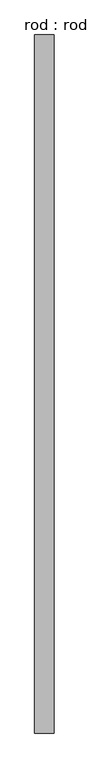
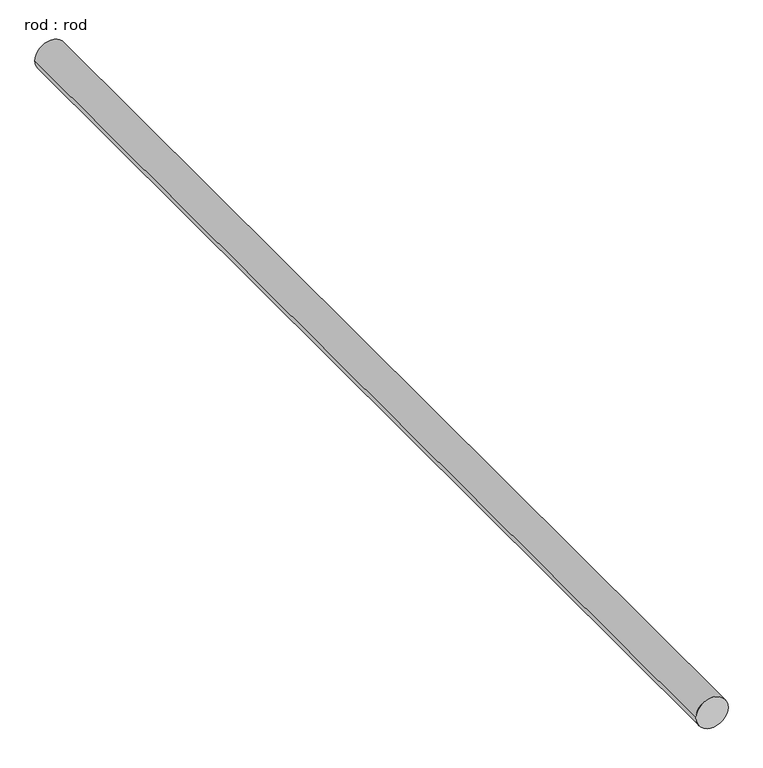
"""IFC4 building model written with IfcOpenShell, lengths in millimetres: proxy geometry, rod : rod."""

import ifcopenshell
import ifcopenshell.guid

model = None  # the IFC model being written
_history = None  # IfcOwnerHistory: only IFC2X3 demands one
_inside = {}  # id of a spatial element -> (the spatial element, [elements in it])
_under = {}  # id of a project, library or spatial element -> (it, [spatial elements below it])
_declared = {}  # id of a project -> (the project, [libraries it declares])
_typed = {}  # id of a type object -> (the type object, [elements of that type])
_made_of = {}  # id of a material, layer set ... -> (it, [elements and type objects made of it])


def new_model(schema):
    """Start an empty IFC model of exactly this schema.

    Asked for "IFC4X3", IfcOpenShell would pick the latest addendum, in which some entities
    have other attributes; the version numbers below select the first issue.
    IFC2X3 requires an IfcOwnerHistory on every rooted entity: one is made here for all.
    """
    global model, _history
    if schema == "IFC4X3":
        model = ifcopenshell.file(schema_version=(4, 3, 0, 0))
    else:
        model = ifcopenshell.file(schema=schema)
    _inside.clear()
    _under.clear()
    _declared.clear()
    _typed.clear()
    _made_of.clear()
    _history = None
    if model.schema == "IFC2X3":
        org = make("IfcOrganization", Name="unknown")
        user = make(
            "IfcPersonAndOrganization",
            ThePerson=make("IfcPerson", FamilyName="unknown"),
            TheOrganization=org,
        )
        app = make(
            "IfcApplication",
            ApplicationDeveloper=org,
            Version="unknown",
            ApplicationFullName="unknown",
            ApplicationIdentifier="unknown",
        )
        _history = make(
            "IfcOwnerHistory",
            OwningUser=user,
            OwningApplication=app,
            ChangeAction="ADDED",
            CreationDate=0,
        )
    return model


def make(cls, **values):
    """One entity of the class cls with the attributes given. An attribute that is None is left unset."""
    return model.create_entity(
        cls, **{name: value for name, value in values.items() if value is not None}
    )


def rooted(cls, **values):
    """An entity with a GlobalId (a new one), such as an element, a storey or a relation."""
    return make(cls, GlobalId=ifcopenshell.guid.new(), OwnerHistory=_history, **values)


def si_unit(unit_type, name, prefix=None):
    """IfcSIUnit, for example si_unit("LENGTHUNIT", "METRE", prefix="MILLI")."""
    return make("IfcSIUnit", UnitType=unit_type, Prefix=prefix, Name=name)


def assignment(units):
    """IfcUnitAssignment: the units of a project."""
    return None if units is None else make("IfcUnitAssignment", Units=units)


def point(xyz):
    """IfcCartesianPoint."""
    return None if xyz is None else make("IfcCartesianPoint", Coordinates=xyz)


def direction(xyz):
    """IfcDirection."""
    return None if xyz is None else make("IfcDirection", DirectionRatios=xyz)


def frame(location, z_axis=None, x_axis=None):
    """IfcAxis2Placement3D, a coordinate frame: its origin and axes. An axis left out is left unset."""
    return make(
        "IfcAxis2Placement3D",
        Location=point(location),
        Axis=direction(z_axis),
        RefDirection=direction(x_axis),
    )


def frame_2d(location, x_axis=None):
    """IfcAxis2Placement2D, a coordinate frame in the plane: its origin and x axis."""
    return make(
        "IfcAxis2Placement2D", Location=point(location), RefDirection=direction(x_axis)
    )


def origin():
    """The frame at (0, 0, 0) with its axes left unset."""
    return frame((0.0, 0.0, 0.0))


def place(relative_to, where):
    """IfcLocalPlacement: puts the frame where relative to a parent placement (None: the world)."""
    return make(
        "IfcLocalPlacement", PlacementRelTo=relative_to, RelativePlacement=where
    )


def context(
    kind, dimensions, precision=None, world=None, true_north=None, identifier=None
):
    """IfcGeometricRepresentationContext, for example the 3D "Model" context."""
    return make(
        "IfcGeometricRepresentationContext",
        ContextIdentifier=identifier,
        ContextType=kind,
        CoordinateSpaceDimension=dimensions,
        Precision=precision,
        WorldCoordinateSystem=world,
        TrueNorth=true_north,
    )


def project(units=None, contexts=None):
    """IfcProject with its units and contexts."""
    return rooted(
        "IfcProject",
        Name="project",
        RepresentationContexts=contexts,
        UnitsInContext=assignment(units),
    )


def spatial(cls, under=None, at=None, **own):
    """A site, building, storey or space (cls), placed at a placement, below another one or the project."""
    s = rooted(cls, ObjectPlacement=at, **own)
    if under is not None:
        _under.setdefault(under.id(), (under, []))[1].append(s)
    return s


def circle_curve(where, radius):
    """IfcCircle in the frame where."""
    return make("IfcCircle", Position=where, Radius=radius)


def trimmed(basis, trim1, trim2, sense, master):
    """IfcTrimmedCurve: the piece of a basis curve between two trims."""
    return make(
        "IfcTrimmedCurve",
        BasisCurve=basis,
        Trim1=trim1,
        Trim2=trim2,
        SenseAgreement=sense,
        MasterRepresentation=master,
    )


def segment(curve, same_sense, transition):
    """IfcCompositeCurveSegment."""
    return make(
        "IfcCompositeCurveSegment",
        Transition=transition,
        SameSense=same_sense,
        ParentCurve=curve,
    )


def composite_curve(segments, self_intersect=None):
    """IfcCompositeCurve: segments joined end to end."""
    return make("IfcCompositeCurve", Segments=segments, SelfIntersect=self_intersect)


def outline(outer, holes=None, kind="AREA"):
    """IfcArbitraryClosedProfileDef: a profile drawn as a closed curve; with holes, ...WithVoids."""
    if holes is None:
        return make("IfcArbitraryClosedProfileDef", ProfileType=kind, OuterCurve=outer)
    return make(
        "IfcArbitraryProfileDefWithVoids",
        ProfileType=kind,
        OuterCurve=outer,
        InnerCurves=holes,
    )


def extrude(swept, where, along, depth):
    """IfcExtrudedAreaSolid: the profile swept, set in the frame where, extruded along a direction by depth."""
    return make(
        "IfcExtrudedAreaSolid",
        SweptArea=swept,
        Position=where,
        ExtrudedDirection=direction(along),
        Depth=depth,
    )


def shape(context_of_items, identifier, shape_type, items):
    """IfcShapeRepresentation: the items that make up one representation, for example the "Body"."""
    return make(
        "IfcShapeRepresentation",
        ContextOfItems=context_of_items,
        RepresentationIdentifier=identifier,
        RepresentationType=shape_type,
        Items=items,
    )


def source(mapping_origin, context_of_items, identifier, shape_type, items):
    """IfcRepresentationMap: a shape defined once, which mapped items show again and again."""
    return make(
        "IfcRepresentationMap",
        MappingOrigin=mapping_origin,
        MappedRepresentation=shape(context_of_items, identifier, shape_type, items),
    )


def transform(
    local_origin,
    x_axis=None,
    y_axis=None,
    z_axis=None,
    scale=None,
    scale2=None,
    scale3=None,
    uniform=True,
):
    """IfcCartesianTransformationOperator3D, or its non-uniform kind. x_axis, y_axis, z_axis: its Axis1, 2, 3."""
    if uniform:
        return make(
            "IfcCartesianTransformationOperator3D",
            Axis1=direction(x_axis),
            Axis2=direction(y_axis),
            LocalOrigin=point(local_origin),
            Scale=scale,
            Axis3=direction(z_axis),
        )
    return make(
        "IfcCartesianTransformationOperator3DnonUniform",
        Axis1=direction(x_axis),
        Axis2=direction(y_axis),
        LocalOrigin=point(local_origin),
        Scale=scale,
        Axis3=direction(z_axis),
        Scale2=scale2,
        Scale3=scale3,
    )


def mapped(mapping_source, mapping_target):
    """IfcMappedItem: shows the shape of a source again, moved by a transform."""
    return make(
        "IfcMappedItem", MappingSource=mapping_source, MappingTarget=mapping_target
    )


def made_of(thing, what):
    """Note that an element or type object is made of a material, layer set ...; save() writes the relation."""
    if what is not None:
        _made_of.setdefault(what.id(), (what, []))[1].append(thing)
    return thing


def element(
    cls,
    number,
    at=None,
    inside=None,
    cuts=None,
    type_object=None,
    material=None,
    context=None,
    identifier="Body",
    shape_type=None,
    held_by="IfcProductDefinitionShape",
    body=None,
    shapes=None,
    **own,
):
    """One element of the class cls, such as IfcWall. Its Tag is "e" and its number.

    at: its placement. inside: the storey or other place that contains it. cuts: it is an
    opening in that element (IfcRelVoidsElement). A single representation is given by context,
    identifier, shape_type and body (its items); several are given by shapes. held_by: the class
    of the entity that holds the representations. save() writes the other relations.
    """
    e = rooted(cls, Tag="e%d" % number, ObjectPlacement=at, **own)
    if body is not None:
        shapes = [shape(context, identifier, shape_type, body)]
    if shapes is not None:
        e.Representation = make(held_by, Representations=shapes)
    if inside is not None:
        _inside.setdefault(inside.id(), (inside, []))[1].append(e)
    if cuts is not None:
        rooted(
            "IfcRelVoidsElement", RelatingBuildingElement=cuts, RelatedOpeningElement=e
        )
    if type_object is not None:
        _typed.setdefault(type_object.id(), (type_object, []))[1].append(e)
    return made_of(e, material)


def aggregate(whole, parts):
    """IfcRelAggregates: a whole, such as a stair, and the parts it consists of."""
    return rooted("IfcRelAggregates", RelatingObject=whole, RelatedObjects=parts)


def save(model, path):
    """Write the relations noted so far, then the file.

    IfcRelAggregates (storeys below a building ...), IfcRelContainedInSpatialStructure (elements
    in a storey), IfcRelDefinesByType, IfcRelAssociatesMaterial and IfcRelDeclares: one each for
    every whole, place, type object, material and project.
    """
    for whole, parts in _under.values():
        aggregate(whole, parts)
    for where, things in _inside.values():
        rooted(
            "IfcRelContainedInSpatialStructure",
            RelatedElements=things,
            RelatingStructure=where,
        )
    for kind, things in _typed.values():
        rooted("IfcRelDefinesByType", RelatedObjects=things, RelatingType=kind)
    for what, things in _made_of.values():
        rooted("IfcRelAssociatesMaterial", RelatedObjects=things, RelatingMaterial=what)
    for by, libraries in _declared.values():
        rooted("IfcRelDeclares", RelatingContext=by, RelatedDefinitions=libraries)
    model.write(path)


def rod_rod_39824f73(model_context):
    return source(origin(), model_context, "Body", "SweptSolid", [
        extrude(outline(composite_curve([segment(trimmed(circle_curve(frame_2d((0.0108462, 0.0)), 200.0), [point((0.0108462, 200.0))], [point((0.0108462, -200.0))], False, "CARTESIAN"), True, "CONTINUOUS"), segment(trimmed(circle_curve(frame_2d((0.0108462, 0.0)), 200.0), [point((0.0108462, -200.0))], [point((0.0108462, 200.0))], False, "CARTESIAN"), True, "CONTINUOUS")], self_intersect=False)), frame((0.0, -3046.1602736, 0.0), z_axis=(0.0, 1.0, 0.0), x_axis=(0.0, 0.0, 1.0)), (0.0, 0.0, 1.0), 14277.7777778),
    ])


if __name__ == "__main__":
    model = new_model("IFC4")
    model_context = context("Model", 3, world=origin())
    ifc_project = project(units=[si_unit("LENGTHUNIT", "METRE", prefix="MILLI")], contexts=[model_context])
    site = spatial("IfcSite", under=ifc_project)
    building = spatial("IfcBuilding", under=site)
    placement = place(None, origin())
    rod_rod_shape = rod_rod_39824f73(model_context)
    element("IfcBuildingElementProxy", 1, Name="rod : rod", ObjectType="rod : rod", at=placement, inside=building, context=model_context, shape_type="MappedRepresentation", body=[
        mapped(rod_rod_shape, transform((0.0, 0.0, 0.0), x_axis=(1.0, 0.0, 0.0), y_axis=(0.0, 1.0, 0.0), z_axis=(0.0, 0.0, 1.0))),
    ])
    save(model, "model.ifc")

# Revit data of these elements
# Type "rod : rod"
#   Default Elevation = 0
